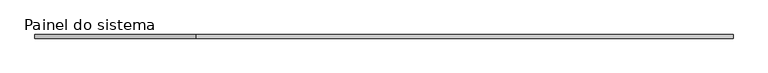
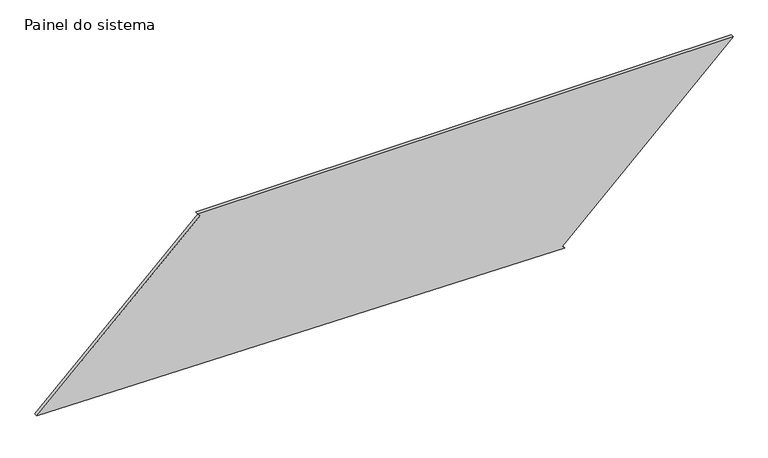
"""IFC4 building model written with IfcOpenShell, lengths in millimetres: plate geometry, Painel do sistema : Envidraçado."""

import ifcopenshell
import ifcopenshell.guid

model = None  # the IFC model being written
_history = None  # IfcOwnerHistory: only IFC2X3 demands one
_inside = {}  # id of a spatial element -> (the spatial element, [elements in it])
_under = {}  # id of a project, library or spatial element -> (it, [spatial elements below it])
_declared = {}  # id of a project -> (the project, [libraries it declares])
_typed = {}  # id of a type object -> (the type object, [elements of that type])
_made_of = {}  # id of a material, layer set ... -> (it, [elements and type objects made of it])


def new_model(schema):
    """Start an empty IFC model of exactly this schema.

    Asked for "IFC4X3", IfcOpenShell would pick the latest addendum, in which some entities
    have other attributes; the version numbers below select the first issue.
    IFC2X3 requires an IfcOwnerHistory on every rooted entity: one is made here for all.
    """
    global model, _history
    if schema == "IFC4X3":
        model = ifcopenshell.file(schema_version=(4, 3, 0, 0))
    else:
        model = ifcopenshell.file(schema=schema)
    _inside.clear()
    _under.clear()
    _declared.clear()
    _typed.clear()
    _made_of.clear()
    _history = None
    if model.schema == "IFC2X3":
        org = make("IfcOrganization", Name="unknown")
        user = make(
            "IfcPersonAndOrganization",
            ThePerson=make("IfcPerson", FamilyName="unknown"),
            TheOrganization=org,
        )
        app = make(
            "IfcApplication",
            ApplicationDeveloper=org,
            Version="unknown",
            ApplicationFullName="unknown",
            ApplicationIdentifier="unknown",
        )
        _history = make(
            "IfcOwnerHistory",
            OwningUser=user,
            OwningApplication=app,
            ChangeAction="ADDED",
            CreationDate=0,
        )
    return model


def make(cls, **values):
    """One entity of the class cls with the attributes given. An attribute that is None is left unset."""
    return model.create_entity(
        cls, **{name: value for name, value in values.items() if value is not None}
    )


def rooted(cls, **values):
    """An entity with a GlobalId (a new one), such as an element, a storey or a relation."""
    return make(cls, GlobalId=ifcopenshell.guid.new(), OwnerHistory=_history, **values)


def si_unit(unit_type, name, prefix=None):
    """IfcSIUnit, for example si_unit("LENGTHUNIT", "METRE", prefix="MILLI")."""
    return make("IfcSIUnit", UnitType=unit_type, Prefix=prefix, Name=name)


def assignment(units):
    """IfcUnitAssignment: the units of a project."""
    return None if units is None else make("IfcUnitAssignment", Units=units)


def point(xyz):
    """IfcCartesianPoint."""
    return None if xyz is None else make("IfcCartesianPoint", Coordinates=xyz)


def direction(xyz):
    """IfcDirection."""
    return None if xyz is None else make("IfcDirection", DirectionRatios=xyz)


def frame(location, z_axis=None, x_axis=None):
    """IfcAxis2Placement3D, a coordinate frame: its origin and axes. An axis left out is left unset."""
    return make(
        "IfcAxis2Placement3D",
        Location=point(location),
        Axis=direction(z_axis),
        RefDirection=direction(x_axis),
    )


def origin():
    """The frame at (0, 0, 0) with its axes left unset."""
    return frame((0.0, 0.0, 0.0))


def place(relative_to, where):
    """IfcLocalPlacement: puts the frame where relative to a parent placement (None: the world)."""
    return make(
        "IfcLocalPlacement", PlacementRelTo=relative_to, RelativePlacement=where
    )


def context(
    kind, dimensions, precision=None, world=None, true_north=None, identifier=None
):
    """IfcGeometricRepresentationContext, for example the 3D "Model" context."""
    return make(
        "IfcGeometricRepresentationContext",
        ContextIdentifier=identifier,
        ContextType=kind,
        CoordinateSpaceDimension=dimensions,
        Precision=precision,
        WorldCoordinateSystem=world,
        TrueNorth=true_north,
    )


def project(units=None, contexts=None):
    """IfcProject with its units and contexts."""
    return rooted(
        "IfcProject",
        Name="project",
        RepresentationContexts=contexts,
        UnitsInContext=assignment(units),
    )


def spatial(cls, under=None, at=None, **own):
    """A site, building, storey or space (cls), placed at a placement, below another one or the project."""
    s = rooted(cls, ObjectPlacement=at, **own)
    if under is not None:
        _under.setdefault(under.id(), (under, []))[1].append(s)
    return s


def polyline(points):
    """IfcPolyline through the points."""
    return make("IfcPolyline", Points=[point(p) for p in points])


def outline(outer, holes=None, kind="AREA"):
    """IfcArbitraryClosedProfileDef: a profile drawn as a closed curve; with holes, ...WithVoids."""
    if holes is None:
        return make("IfcArbitraryClosedProfileDef", ProfileType=kind, OuterCurve=outer)
    return make(
        "IfcArbitraryProfileDefWithVoids",
        ProfileType=kind,
        OuterCurve=outer,
        InnerCurves=holes,
    )


def extrude(swept, where, along, depth):
    """IfcExtrudedAreaSolid: the profile swept, set in the frame where, extruded along a direction by depth."""
    return make(
        "IfcExtrudedAreaSolid",
        SweptArea=swept,
        Position=where,
        ExtrudedDirection=direction(along),
        Depth=depth,
    )


def shape(context_of_items, identifier, shape_type, items):
    """IfcShapeRepresentation: the items that make up one representation, for example the "Body"."""
    return make(
        "IfcShapeRepresentation",
        ContextOfItems=context_of_items,
        RepresentationIdentifier=identifier,
        RepresentationType=shape_type,
        Items=items,
    )


def source(mapping_origin, context_of_items, identifier, shape_type, items):
    """IfcRepresentationMap: a shape defined once, which mapped items show again and again."""
    return make(
        "IfcRepresentationMap",
        MappingOrigin=mapping_origin,
        MappedRepresentation=shape(context_of_items, identifier, shape_type, items),
    )


def transform(
    local_origin,
    x_axis=None,
    y_axis=None,
    z_axis=None,
    scale=None,
    scale2=None,
    scale3=None,
    uniform=True,
):
    """IfcCartesianTransformationOperator3D, or its non-uniform kind. x_axis, y_axis, z_axis: its Axis1, 2, 3."""
    if uniform:
        return make(
            "IfcCartesianTransformationOperator3D",
            Axis1=direction(x_axis),
            Axis2=direction(y_axis),
            LocalOrigin=point(local_origin),
            Scale=scale,
            Axis3=direction(z_axis),
        )
    return make(
        "IfcCartesianTransformationOperator3DnonUniform",
        Axis1=direction(x_axis),
        Axis2=direction(y_axis),
        LocalOrigin=point(local_origin),
        Scale=scale,
        Axis3=direction(z_axis),
        Scale2=scale2,
        Scale3=scale3,
    )


def mapped(mapping_source, mapping_target):
    """IfcMappedItem: shows the shape of a source again, moved by a transform."""
    return make(
        "IfcMappedItem", MappingSource=mapping_source, MappingTarget=mapping_target
    )


def made_of(thing, what):
    """Note that an element or type object is made of a material, layer set ...; save() writes the relation."""
    if what is not None:
        _made_of.setdefault(what.id(), (what, []))[1].append(thing)
    return thing


def element(
    cls,
    number,
    at=None,
    inside=None,
    cuts=None,
    type_object=None,
    material=None,
    context=None,
    identifier="Body",
    shape_type=None,
    held_by="IfcProductDefinitionShape",
    body=None,
    shapes=None,
    **own,
):
    """One element of the class cls, such as IfcWall. Its Tag is "e" and its number.

    at: its placement. inside: the storey or other place that contains it. cuts: it is an
    opening in that element (IfcRelVoidsElement). A single representation is given by context,
    identifier, shape_type and body (its items); several are given by shapes. held_by: the class
    of the entity that holds the representations. save() writes the other relations.
    """
    e = rooted(cls, Tag="e%d" % number, ObjectPlacement=at, **own)
    if body is not None:
        shapes = [shape(context, identifier, shape_type, body)]
    if shapes is not None:
        e.Representation = make(held_by, Representations=shapes)
    if inside is not None:
        _inside.setdefault(inside.id(), (inside, []))[1].append(e)
    if cuts is not None:
        rooted(
            "IfcRelVoidsElement", RelatingBuildingElement=cuts, RelatedOpeningElement=e
        )
    if type_object is not None:
        _typed.setdefault(type_object.id(), (type_object, []))[1].append(e)
    return made_of(e, material)


def aggregate(whole, parts):
    """IfcRelAggregates: a whole, such as a stair, and the parts it consists of."""
    return rooted("IfcRelAggregates", RelatingObject=whole, RelatedObjects=parts)


def save(model, path):
    """Write the relations noted so far, then the file.

    IfcRelAggregates (storeys below a building ...), IfcRelContainedInSpatialStructure (elements
    in a storey), IfcRelDefinesByType, IfcRelAssociatesMaterial and IfcRelDeclares: one each for
    every whole, place, type object, material and project.
    """
    for whole, parts in _under.values():
        aggregate(whole, parts)
    for where, things in _inside.values():
        rooted(
            "IfcRelContainedInSpatialStructure",
            RelatedElements=things,
            RelatingStructure=where,
        )
    for kind, things in _typed.values():
        rooted("IfcRelDefinesByType", RelatedObjects=things, RelatingType=kind)
    for what, things in _made_of.values():
        rooted("IfcRelAssociatesMaterial", RelatedObjects=things, RelatingMaterial=what)
    for by, libraries in _declared.values():
        rooted("IfcRelDeclares", RelatingContext=by, RelatedDefinitions=libraries)
    model.write(path)


def painel_do_sistema_01f7b47b(model_context):
    return source(origin(), model_context, "Body", "SweptSolid", [
        extrude(outline(polyline([(0.0, 1242.7103806), (18.146416, 1225.5142302), (1138.363193, 2407.6345988), (1138.363193, -1296.1434032), (1120.2167771, -1278.9472528), (50.6349184, -2407.6345988), (0.0, 1242.7103806)])), frame((0.0, 24.5, 0.0), z_axis=(0.0, 1.0, 0.0), x_axis=(0.0, 0.0, 1.0)), (0.0, 0.0, 1.0), 25.0),
    ])


if __name__ == "__main__":
    model = new_model("IFC4")
    model_context = context("Model", 3, world=origin())
    ifc_project = project(units=[si_unit("LENGTHUNIT", "METRE", prefix="MILLI")], contexts=[model_context])
    site = spatial("IfcSite", under=ifc_project)
    building = spatial("IfcBuilding", under=site)
    placement = place(None, origin())
    painel_do_sistema_shape = painel_do_sistema_01f7b47b(model_context)
    element("IfcPlate", 1, ObjectType="Painel do sistema : Envidraçado", at=placement, inside=building, context=model_context, shape_type="MappedRepresentation", body=[
        mapped(painel_do_sistema_shape, transform((0.0, 0.0, 0.0), x_axis=(1.0, 0.0, 0.0), y_axis=(0.0, 1.0, 0.0), z_axis=(0.0, 0.0, 1.0))),
    ])
    save(model, "model.ifc")

# Revit data of these elements
# Type "Painel do sistema : Envidraçado"
#   Construction Type Id = "GSP4R"
#   Analytic Construction = "Vidraça única Pilkington 1/8 pol"
#   Visual Light Transmittance = 0.9
#   Solar Heat Gain Coefficient = 0.86
#   Heat Transfer Coefficient (U) = 6.7069 W/(m²·K)
# Element 1 (IfcPlate, "Painel do sistema : Envidraçado")
#   Materials on its faces: "Vidro"
# Materials
#   "Vidro": class "Vidro", colour RGB 0 128 192, transparency 0.9, Description = "Vidro de sílica", Cost = 0
